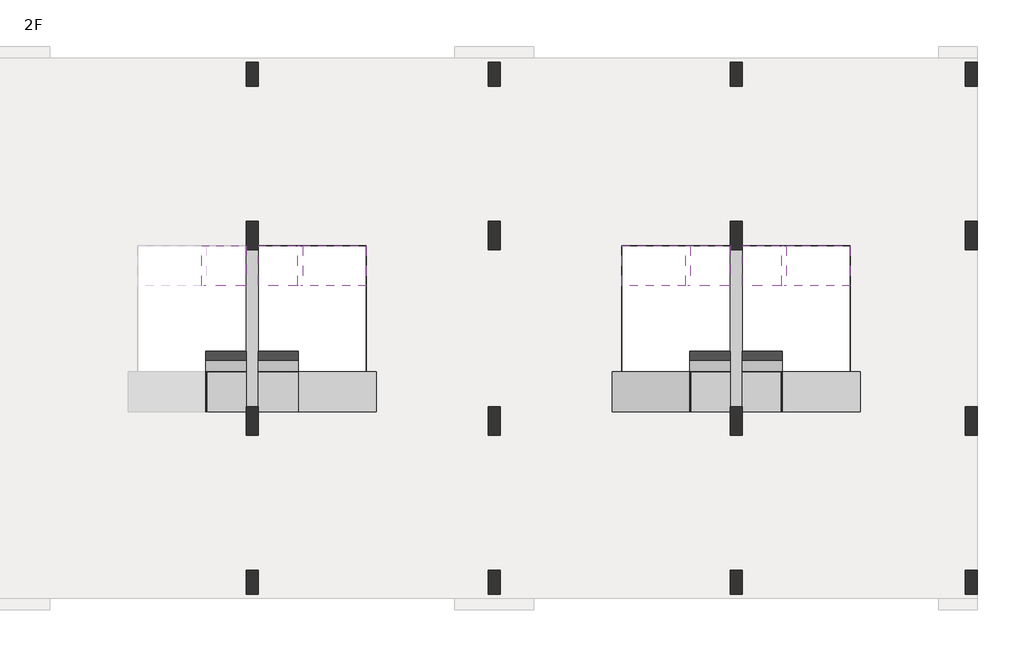
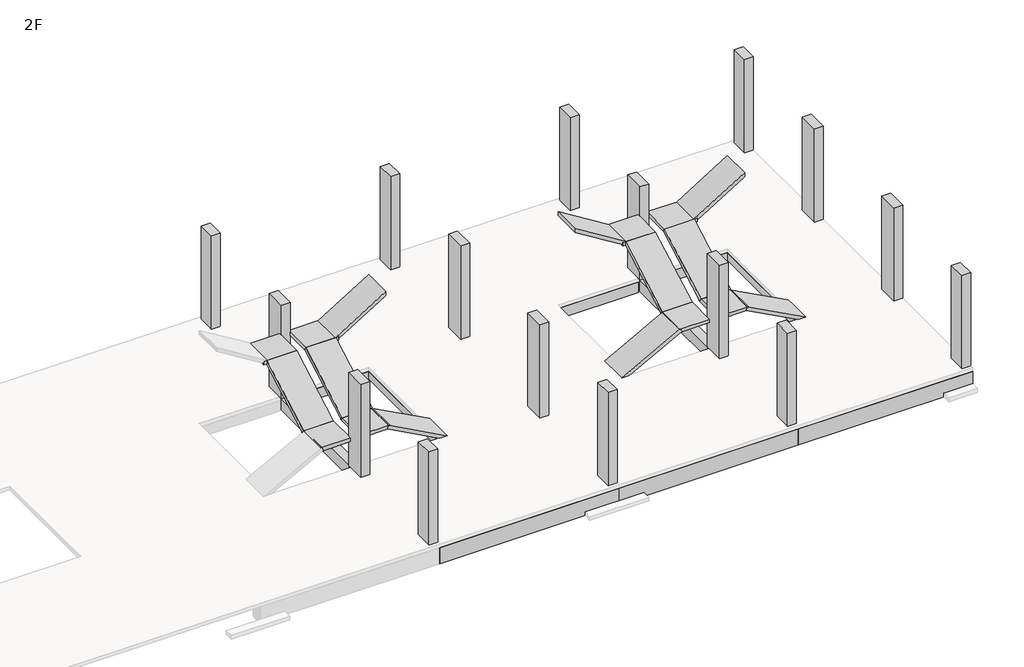
# One storey, part 2 of 2: 45 beams, 16 columns.
"""IFC4 building model written with IfcOpenShell, lengths in millimetres."""

from ifc_helpers import new_model, si_unit, frame, origin, place, context, project, spatial, polyline, outline, extrude, faceted_brep, element, save

model = new_model("IFC4")

# Units and contexts
model_context = context("Model", 3, world=origin())
ifc_project = project(units=[si_unit("LENGTHUNIT", "METRE", prefix="MILLI")], contexts=[model_context])

# Site, building, storey
site = spatial("IfcSite", under=ifc_project)
building = spatial("IfcBuilding", under=site)
storey = spatial("IfcBuildingStorey", under=building, Name="2F", Elevation=4030.0)

# Beams
placement = place(None, origin())
element("IfcBeam", 1, ObjectType="M_Concrete-Rectangular Beam : 1000x120", at=placement, inside=storey, context=model_context, shape_type="Brep", body=[
    faceted_brep([(16700.0000058, 7550.0000002, 6280.0), (17700.0000058, 7550.0000002, 6280.0), (17700.0000058, 7609.0063595, 6175.5095719), (16700.0000058, 7609.0063595, 6175.5095719), (16700.0000058, 5424.9999998, 5080.0), (16700.0000058, 5484.0063591, 4975.5095719), (17700.0000058, 5484.0063591, 4975.5095719), (17700.0000058, 5424.9999998, 5080.0), (17700.0000058, 5524.9999998, 4998.6589219), (17700.0000058, 7581.5414925, 6160.0), (16700.0000058, 5524.9999998, 4998.6589219), (16700.0000058, 7581.5414925, 6160.0)], [[[0, 1, 2, 3]], [[4, 5, 6, 7]], [[1, 0, 4, 7]], [[2, 1, 7, 6, 8, 9]], [[3, 2, 9, 8, 6, 5, 10, 11]], [[0, 3, 11, 10, 5, 4]]]),
])
element("IfcBeam", 2, ObjectType="M_Concrete-Rectangular Beam : 1000x120", at=placement, inside=storey, context=model_context, shape_type="Brep", body=[
    faceted_brep([(16600.0000058, 7550.0000002, 6280.0), (16600.0000058, 8550.0000002, 6280.0), (16600.0000058, 8550.0000002, 6160.0), (16600.0000058, 7550.0000002, 6160.0), (17700.0000058, 8550.0000002, 6160.0), (17700.0000058, 8550.0000002, 6280.0), (17700.0000058, 7550.0000002, 6280.0), (17700.0000058, 7609.0063595, 6175.5095719), (17700.0000058, 7581.5414925, 6160.0), (16700.0000058, 7550.0000002, 6280.0), (16700.0000058, 7581.5414925, 6160.0), (16700.0000058, 7550.0000002, 6160.0), (16700.0000058, 7609.0063595, 6175.5095719)], [[[0, 1, 2, 3]], [[4, 5, 6, 7, 8]], [[1, 0, 9, 6, 5]], [[2, 1, 5, 4]], [[3, 2, 4, 8, 10, 11]], [[0, 3, 11, 9]], [[12, 7, 6, 9]], [[7, 12, 10, 8]], [[12, 9, 11, 10]]]),
])
element("IfcBeam", 3, ObjectType="M_Concrete-Rectangular Beam : 1000x120", at=placement, inside=storey, context=model_context, shape_type="Brep", body=[
    faceted_brep([(17700.0000058, 5524.9999998, 4960.0), (16700.0000058, 5524.9999998, 4960.0), (16700.0000058, 5524.9999998, 4998.6589219), (17700.0000058, 5524.9999998, 4998.6589219), (17700.0000058, 4424.9999998, 4960.0), (17700.0000058, 4424.9999998, 5080.0), (16730.4772117, 4424.9999998, 5080.0), (16787.1330628, 4424.9999998, 4974.2166623), (16760.588832, 4424.9999998, 4960.0), (17700.0000058, 5424.9999998, 5080.0), (16700.0000058, 5424.9999998, 5080.0), (16700.0000058, 4424.9999998, 5080.0), (17700.0000058, 5484.0063591, 4975.5095719), (16760.588832, 5424.9999998, 4960.0), (16700.0000058, 5424.9999998, 4960.0), (16700.0000058, 4424.9999998, 5063.6768996), (16700.0000058, 5484.0063591, 4975.5095719), (16700.0000058, 5424.9999998, 5063.6768996), (16730.4772117, 5424.9999998, 5080.0), (16787.1330628, 5424.9999998, 4974.2166623)], [[[0, 1, 2, 3]], [[4, 5, 6, 7, 8]], [[6, 5, 9, 10, 11]], [[5, 4, 0, 3, 12, 9]], [[1, 0, 4, 8, 13, 14]], [[15, 11, 10, 16, 2, 1, 14, 17]], [[6, 18, 19, 7]], [[18, 6, 15, 17]], [[7, 19, 13, 8]], [[19, 18, 17, 14, 13]], [[11, 15, 6]], [[12, 16, 10, 9]], [[16, 12, 3, 2]]]),
])
element("IfcBeam", 4, ObjectType="M_Concrete-Rectangular Beam : 1000x120", at=placement, inside=storey, context=model_context, shape_type="Brep", body=[
    faceted_brep([(18969.5227998, 4424.9999998, 5080.0), (18969.5227998, 5424.9999998, 5080.0), (18912.8669488, 5424.9999998, 4974.2166623), (18912.8669488, 4424.9999998, 4974.2166623), (19000.0000058, 4424.9999998, 5063.6768996), (20930.0000065, 4424.9999998, 4030.0), (20930.0000065, 5424.9999998, 4030.0), (19000.0000058, 5424.9999998, 5063.6768996), (18939.4111796, 4424.9999998, 4960.0), (20675.8338483, 4424.9999998, 4030.0), (18939.4111796, 5424.9999998, 4960.0), (20680.0000058, 5424.9999998, 4027.7686732), (20680.0000058, 4449.9999998, 4027.7686732), (20675.8338483, 4449.9999998, 4030.0), (20680.0000058, 5424.9999998, 4030.0), (20680.0000058, 4449.9999998, 4030.0)], [[[0, 1, 2, 3]], [[1, 0, 4, 5, 6, 7]], [[0, 3, 8, 9, 5, 4]], [[3, 2, 10, 11, 12, 13, 9, 8]], [[2, 1, 7, 6, 14, 11, 10]], [[14, 6, 5, 9, 13, 15]], [[11, 14, 15, 12]], [[15, 13, 12]]]),
])
element("IfcBeam", 5, ObjectType="M_Concrete-Rectangular Beam : 1000x120", at=placement, inside=storey, context=model_context, shape_type="Brep", body=[
    faceted_brep([(19000.0000058, 7550.0000002, 6280.0), (19000.0000058, 7609.0063595, 6175.5095719), (18000.0000058, 7609.0063595, 6175.5095719), (18000.0000058, 7550.0000002, 6280.0), (19000.0000058, 5424.9999998, 5080.0), (18000.0000058, 5424.9999998, 5080.0), (18000.0000058, 5484.0063591, 4975.5095719), (19000.0000058, 5484.0063591, 4975.5095719), (18000.0000058, 7581.5414925, 6160.0), (18000.0000058, 5524.9999998, 4998.6589219), (19000.0000058, 7581.5414925, 6160.0), (19000.0000058, 5524.9999998, 4998.6589219)], [[[0, 1, 2, 3]], [[4, 5, 6, 7]], [[3, 5, 4, 0]], [[2, 8, 9, 6, 5, 3]], [[1, 10, 11, 7, 6, 9, 8, 2]], [[0, 4, 7, 11, 10, 1]]]),
])
element("IfcBeam", 6, ObjectType="M_Concrete-Rectangular Beam : 1000x120", at=placement, inside=storey, context=model_context, shape_type="Brep", body=[
    faceted_brep([(19100.0000058, 8550.0000002, 6280.0), (19100.0000058, 7550.0000002, 6280.0), (19100.0000058, 7550.0000002, 6160.0), (19100.0000058, 8550.0000002, 6160.0), (18000.0000058, 8550.0000002, 6280.0), (18000.0000058, 8550.0000002, 6160.0), (18000.0000058, 7581.5414925, 6160.0), (18000.0000058, 7609.0063595, 6175.5095719), (18000.0000058, 7550.0000002, 6280.0), (19000.0000058, 7550.0000002, 6280.0), (19000.0000058, 7550.0000002, 6160.0), (19000.0000058, 7581.5414925, 6160.0), (19000.0000058, 7609.0063595, 6175.5095719)], [[[0, 1, 2, 3]], [[4, 5, 6, 7, 8]], [[1, 0, 4, 8, 9]], [[0, 3, 5, 4]], [[3, 2, 10, 11, 6, 5]], [[2, 1, 9, 10]], [[12, 9, 8, 7]], [[12, 7, 6, 11]], [[9, 12, 11, 10]]]),
])
element("IfcBeam", 7, ObjectType="M_Concrete-Rectangular Beam : 1000x120", at=placement, inside=storey, context=model_context, shape_type="Brep", body=[
    faceted_brep([(18984.2496976, 7549.9999993, 6280.0), (20680.0000464, 7549.9999993, 7330.0), (20680.0000058, 8549.9999993, 7329.9999748), (18984.2496976, 8549.9999993, 6280.0), (20680.0000058, 8549.9999993, 7188.8582241), (19100.0000058, 8549.9999993, 6210.5302519), (19100.0000058, 8549.9999993, 6280.0), (19100.0000058, 7549.9999993, 6210.5302519), (20680.0000058, 7549.9999993, 7188.8582241), (19000.0000058, 7549.9999993, 6280.0), (19100.0000058, 7549.9999993, 6280.0)], [[[0, 1, 2, 3]], [[3, 2, 4, 5, 6]], [[7, 5, 4, 8]], [[1, 0, 9, 10, 7, 8]], [[10, 6, 5, 7]], [[6, 10, 9, 0, 3]], [[2, 1, 8, 4]]]),
])
element("IfcBeam", 8, ObjectType="M_Concrete-Rectangular Beam : 1000x120", at=placement, inside=storey, context=model_context, shape_type="Brep", body=[
    faceted_brep([(19000.0000058, 5524.9999998, 4960.0), (18000.0000058, 5524.9999998, 4960.0), (18000.0000058, 5524.9999998, 4998.6589219), (19000.0000058, 5524.9999998, 4998.6589219), (18000.0000058, 4424.9999998, 5080.0), (18000.0000058, 4424.9999998, 4960.0), (18939.4111796, 4424.9999998, 4960.0), (18912.8669488, 4424.9999998, 4974.2166623), (18969.5227998, 4424.9999998, 5080.0), (19000.0000058, 4424.9999998, 5080.0), (19000.0000058, 5424.9999998, 5080.0), (18000.0000058, 5424.9999998, 5080.0), (18000.0000058, 5484.0063591, 4975.5095719), (19000.0000058, 5424.9999998, 4960.0), (18939.4111796, 5424.9999998, 4960.0), (19000.0000058, 4424.9999998, 5063.6768996), (19000.0000058, 5424.9999998, 5063.6768996), (19000.0000058, 5484.0063591, 4975.5095719), (18969.5227998, 5424.9999998, 5080.0), (18912.8669488, 5424.9999998, 4974.2166623)], [[[0, 1, 2, 3]], [[4, 5, 6, 7, 8]], [[8, 9, 10, 11, 4]], [[5, 4, 11, 12, 2, 1]], [[1, 0, 13, 14, 6, 5]], [[9, 15, 16, 13, 0, 3, 17, 10]], [[18, 8, 7, 19]], [[8, 18, 16, 15]], [[19, 7, 6, 14]], [[18, 19, 14, 13, 16]], [[15, 9, 8]], [[17, 12, 11, 10]], [[12, 17, 3, 2]]]),
])
element("IfcBeam", 9, ObjectType="M_Concrete-Rectangular Beam : 1000x120", at=placement, inside=storey, context=model_context, shape_type="Brep", body=[
    faceted_brep([(28730.4772098, 5424.9999998, 5080.0), (28730.4772098, 4424.9999998, 5080.0), (28787.1330609, 4424.9999998, 4974.2166623), (28787.1330609, 5424.9999998, 4974.2166623), (28700.0000039, 5424.9999998, 5063.6768996), (26770.0000031, 5424.9999998, 4030.0), (26770.0000031, 4424.9999998, 4030.0), (28700.0000039, 4424.9999998, 5063.6768996), (27024.1661613, 4424.9999998, 4030.0), (28760.5888301, 4424.9999998, 4960.0), (27024.1661613, 4449.9999998, 4030.0), (27020.000004, 4449.9999998, 4027.7686733), (27020.000004, 5424.9999998, 4027.7686733), (28760.5888301, 5424.9999998, 4960.0), (27020.000004, 5424.9999998, 4030.0), (27020.000004, 4449.9999998, 4030.0)], [[[0, 1, 2, 3]], [[1, 0, 4, 5, 6, 7]], [[2, 1, 7, 6, 8, 9]], [[3, 2, 9, 8, 10, 11, 12, 13]], [[0, 3, 13, 12, 14, 5, 4]], [[5, 14, 15, 10, 8, 6]], [[14, 12, 11, 15]], [[10, 15, 11]]]),
])
element("IfcBeam", 10, ObjectType="M_Concrete-Rectangular Beam : 1000x120", at=placement, inside=storey, context=model_context, shape_type="Brep", body=[
    faceted_brep([(28700.0000039, 7550.0000002, 6280.0), (29700.0000039, 7550.0000002, 6280.0), (29700.0000039, 7609.0063595, 6175.5095719), (28700.0000039, 7609.0063595, 6175.5095719), (28700.0000039, 5424.9999998, 5080.0), (28700.0000039, 5484.0063591, 4975.5095719), (29700.0000039, 5484.0063591, 4975.5095719), (29700.0000039, 5424.9999998, 5080.0), (29700.0000039, 5524.9999998, 4998.6589219), (29700.0000039, 7581.5414925, 6160.0), (28700.0000039, 5524.9999998, 4998.6589219), (28700.0000039, 7581.5414925, 6160.0)], [[[0, 1, 2, 3]], [[4, 5, 6, 7]], [[1, 0, 4, 7]], [[2, 1, 7, 6, 8, 9]], [[3, 2, 9, 8, 6, 5, 10, 11]], [[0, 3, 11, 10, 5, 4]]]),
])
element("IfcBeam", 11, ObjectType="M_Concrete-Rectangular Beam : 1000x120", at=placement, inside=storey, context=model_context, shape_type="Brep", body=[
    faceted_brep([(28600.0000039, 7550.0000002, 6280.0), (28600.0000039, 8550.0000002, 6280.0), (28600.0000039, 8550.0000002, 6160.0), (28600.0000039, 7550.0000002, 6160.0), (29700.0000039, 8550.0000002, 6160.0), (29700.0000039, 8550.0000002, 6280.0), (29700.0000039, 7550.0000002, 6280.0), (29700.0000039, 7609.0063595, 6175.5095719), (29700.0000039, 7581.5414925, 6160.0), (28700.0000039, 7550.0000002, 6280.0), (28700.0000039, 7581.5414925, 6160.0), (28700.0000039, 7550.0000002, 6160.0), (28700.0000039, 7609.0063595, 6175.5095719)], [[[0, 1, 2, 3]], [[4, 5, 6, 7, 8]], [[1, 0, 9, 6, 5]], [[2, 1, 5, 4]], [[3, 2, 4, 8, 10, 11]], [[0, 3, 11, 9]], [[12, 7, 6, 9]], [[7, 12, 10, 8]], [[12, 9, 11, 10]]]),
])
element("IfcBeam", 12, ObjectType="M_Concrete-Rectangular Beam : 1000x120", at=placement, inside=storey, context=model_context, shape_type="Brep", body=[
    faceted_brep([(27019.9999632, 7549.9999993, 7330.0), (28715.750312, 7549.9999993, 6280.0), (28715.750312, 8549.9999993, 6280.0), (27019.9999632, 8549.9999993, 7330.0), (28600.0000039, 8549.9999993, 6280.0), (28600.0000039, 8549.9999993, 6210.5302519), (27020.000004, 8549.9999993, 7188.8582239), (28600.0000039, 7549.9999993, 6210.5302519), (27020.000004, 7549.9999993, 7188.8582239), (28600.0000039, 7549.9999993, 6280.0), (28700.0000039, 7549.9999993, 6280.0)], [[[0, 1, 2, 3]], [[3, 2, 4, 5, 6]], [[5, 7, 8, 6]], [[1, 0, 8, 7, 9, 10]], [[4, 9, 7, 5]], [[9, 4, 2, 1, 10]], [[0, 3, 6, 8]]]),
])
element("IfcBeam", 13, ObjectType="M_Concrete-Rectangular Beam : 1000x120", at=placement, inside=storey, context=model_context, shape_type="Brep", body=[
    faceted_brep([(29700.0000039, 5524.9999998, 4960.0), (28700.0000039, 5524.9999998, 4960.0), (28700.0000039, 5524.9999998, 4998.6589219), (29700.0000039, 5524.9999998, 4998.6589219), (29700.0000039, 4424.9999998, 4960.0), (29700.0000039, 4424.9999998, 5080.0), (28730.4772098, 4424.9999998, 5080.0), (28787.1330609, 4424.9999998, 4974.2166623), (28760.5888301, 4424.9999998, 4960.0), (29700.0000039, 5424.9999998, 5080.0), (28700.0000039, 5424.9999998, 5080.0), (28700.0000039, 4424.9999998, 5080.0), (29700.0000039, 5484.0063591, 4975.5095719), (28760.5888301, 5424.9999998, 4960.0), (28700.0000039, 5424.9999998, 4960.0), (28700.0000039, 4424.9999998, 5063.6768996), (28700.0000039, 5484.0063591, 4975.5095719), (28700.0000039, 5424.9999998, 5063.6768996), (28730.4772098, 5424.9999998, 5080.0), (28787.1330609, 5424.9999998, 4974.2166623)], [[[0, 1, 2, 3]], [[4, 5, 6, 7, 8]], [[6, 5, 9, 10, 11]], [[5, 4, 0, 3, 12, 9]], [[1, 0, 4, 8, 13, 14]], [[15, 11, 10, 16, 2, 1, 14, 17]], [[6, 18, 19, 7]], [[18, 6, 15, 17]], [[7, 19, 13, 8]], [[19, 18, 17, 14, 13]], [[11, 15, 6]], [[12, 16, 10, 9]], [[16, 12, 3, 2]]]),
])
element("IfcBeam", 14, ObjectType="M_Concrete-Rectangular Beam : 1000x120", at=placement, inside=storey, context=model_context, shape_type="Brep", body=[
    faceted_brep([(30969.5227979, 4424.9999998, 5080.0), (30969.5227979, 5424.9999998, 5080.0), (30912.8669468, 5424.9999998, 4974.2166623), (30912.8669468, 4424.9999998, 4974.2166623), (31000.0000039, 4424.9999998, 5063.6768996), (32930.0000046, 4424.9999998, 4030.0), (32930.0000046, 5424.9999998, 4030.0), (31000.0000039, 5424.9999998, 5063.6768996), (30939.4111776, 4424.9999998, 4960.0), (32675.8338464, 4424.9999998, 4030.0), (30939.4111776, 5424.9999998, 4960.0), (32680.0000108, 5424.9999998, 4027.7686695), (32680.0000108, 4449.9999998, 4027.7686695), (32675.8338464, 4449.9999998, 4030.0), (32680.0000108, 5424.9999998, 4030.0), (32680.0000108, 4449.9999998, 4030.0)], [[[0, 1, 2, 3]], [[1, 0, 4, 5, 6, 7]], [[0, 3, 8, 9, 5, 4]], [[3, 2, 10, 11, 12, 13, 9, 8]], [[2, 1, 7, 6, 14, 11, 10]], [[14, 6, 5, 9, 13, 15]], [[11, 14, 15, 12]], [[15, 13, 12]]]),
])
element("IfcBeam", 15, ObjectType="M_Concrete-Rectangular Beam : 1000x120", at=placement, inside=storey, context=model_context, shape_type="Brep", body=[
    faceted_brep([(31000.0000039, 7550.0000002, 6280.0), (31000.0000039, 7609.0063595, 6175.5095719), (30000.0000039, 7609.0063595, 6175.5095719), (30000.0000039, 7550.0000002, 6280.0), (31000.0000039, 5424.9999998, 5080.0), (30000.0000039, 5424.9999998, 5080.0), (30000.0000039, 5484.0063591, 4975.5095719), (31000.0000039, 5484.0063591, 4975.5095719), (30000.0000039, 7581.5414925, 6160.0), (30000.0000039, 5524.9999998, 4998.6589219), (31000.0000039, 7581.5414925, 6160.0), (31000.0000039, 5524.9999998, 4998.6589219)], [[[0, 1, 2, 3]], [[4, 5, 6, 7]], [[3, 5, 4, 0]], [[2, 8, 9, 6, 5, 3]], [[1, 10, 11, 7, 6, 9, 8, 2]], [[0, 4, 7, 11, 10, 1]]]),
])
element("IfcBeam", 16, ObjectType="M_Concrete-Rectangular Beam : 1000x120", at=placement, inside=storey, context=model_context, shape_type="Brep", body=[
    faceted_brep([(31100.0000039, 8550.0000002, 6280.0), (31100.0000039, 7550.0000002, 6280.0), (31100.0000039, 7550.0000002, 6160.0), (31100.0000039, 8550.0000002, 6160.0), (30000.0000039, 8550.0000002, 6280.0), (30000.0000039, 8550.0000002, 6160.0), (30000.0000039, 7581.5414925, 6160.0), (30000.0000039, 7609.0063595, 6175.5095719), (30000.0000039, 7550.0000002, 6280.0), (31000.0000039, 7550.0000002, 6280.0), (31000.0000039, 7550.0000002, 6160.0), (31000.0000039, 7581.5414925, 6160.0), (31000.0000039, 7609.0063595, 6175.5095719)], [[[0, 1, 2, 3]], [[4, 5, 6, 7, 8]], [[1, 0, 4, 8, 9]], [[0, 3, 5, 4]], [[3, 2, 10, 11, 6, 5]], [[2, 1, 9, 10]], [[12, 9, 8, 7]], [[12, 7, 6, 11]], [[9, 12, 11, 10]]]),
])
element("IfcBeam", 17, ObjectType="M_Concrete-Rectangular Beam : 1000x120", at=placement, inside=storey, context=model_context, shape_type="Brep", body=[
    faceted_brep([(30984.2496957, 7549.9999993, 6280.0), (32680.0000445, 7549.9999993, 7330.0), (32680.0000108, 8549.9999993, 7329.9999791), (30984.2496957, 8549.9999993, 6280.0), (32680.0000108, 8549.9999993, 7188.8582284), (31100.0000039, 8549.9999993, 6210.5302519), (31100.0000039, 8549.9999993, 6280.0), (31100.0000039, 7549.9999993, 6210.5302519), (32680.0000108, 7549.9999993, 7188.8582284), (31000.0000039, 7549.9999993, 6280.0), (31100.0000039, 7549.9999993, 6280.0)], [[[0, 1, 2, 3]], [[3, 2, 4, 5, 6]], [[7, 5, 4, 8]], [[1, 0, 9, 10, 7, 8]], [[10, 6, 5, 7]], [[6, 10, 9, 0, 3]], [[2, 1, 8, 4]]]),
])
element("IfcBeam", 18, ObjectType="M_Concrete-Rectangular Beam : 1000x120", at=placement, inside=storey, context=model_context, shape_type="Brep", body=[
    faceted_brep([(31000.0000039, 5524.9999998, 4960.0), (30000.0000039, 5524.9999998, 4960.0), (30000.0000039, 5524.9999998, 4998.6589219), (31000.0000039, 5524.9999998, 4998.6589219), (30000.0000039, 4424.9999998, 5080.0), (30000.0000039, 4424.9999998, 4960.0), (30939.4111776, 4424.9999998, 4960.0), (30912.8669468, 4424.9999998, 4974.2166623), (30969.5227979, 4424.9999998, 5080.0), (31000.0000039, 4424.9999998, 5080.0), (31000.0000039, 5424.9999998, 5080.0), (30000.0000039, 5424.9999998, 5080.0), (30000.0000039, 5484.0063591, 4975.5095719), (31000.0000039, 5424.9999998, 4960.0), (30939.4111776, 5424.9999998, 4960.0), (31000.0000039, 4424.9999998, 5063.6768996), (31000.0000039, 5424.9999998, 5063.6768996), (31000.0000039, 5484.0063591, 4975.5095719), (30969.5227979, 5424.9999998, 5080.0), (30912.8669468, 5424.9999998, 4974.2166623)], [[[0, 1, 2, 3]], [[4, 5, 6, 7, 8]], [[8, 9, 10, 11, 4]], [[5, 4, 11, 12, 2, 1]], [[1, 0, 13, 14, 6, 5]], [[9, 15, 16, 13, 0, 3, 17, 10]], [[18, 8, 7, 19]], [[8, 18, 16, 15]], [[19, 7, 6, 14]], [[18, 19, 14, 13, 16]], [[15, 9, 8]], [[17, 12, 11, 10]], [[12, 17, 3, 2]]]),
])
element("IfcBeam", 19, ObjectType="M_Concrete-Rectangular Beam : 250x400", at=placement, inside=storey, context=model_context, shape_type="Brep", body=[
    faceted_brep([(32930.0000108, 4449.9999998, 3630.0), (32930.0000108, 8549.9999993, 3630.0), (32930.0000108, 8549.9999993, 3900.0), (32930.0000108, 4449.9999998, 3900.0), (32680.0000108, 8549.9999993, 3630.0), (32680.0000108, 4449.9999998, 3630.0), (32680.0000108, 4449.9999998, 3900.0), (32680.0000108, 8549.9999993, 3900.0), (32680.0000108, 8549.9999993, 3881.8224584)], [[[0, 1, 2, 3]], [[4, 1, 0, 5]], [[4, 5, 6, 7, 8]], [[1, 4, 8, 7, 2]], [[5, 0, 3, 6]], [[3, 2, 7, 6]]]),
])
element("IfcBeam", 20, ObjectType="M_Concrete-Rectangular Beam : 250x400", at=placement, inside=storey, context=model_context, shape_type="Brep", body=[
    faceted_brep([(20680.0000058, 8549.9999993, 3630.0), (20680.0000058, 4449.9999998, 3630.0), (20680.0000058, 4449.9999998, 3900.0), (20680.0000058, 8549.9999993, 3900.0), (20680.0000058, 8549.9999993, 3881.8224534), (20930.0000058, 8549.9999993, 3630.0), (20930.0000058, 4449.9999998, 3630.0), (20930.0000058, 8549.9999993, 3900.0), (20930.0000058, 4449.9999998, 3900.0)], [[[0, 1, 2, 3, 4]], [[0, 5, 6, 1]], [[6, 5, 7, 8]], [[5, 0, 4, 3, 7]], [[1, 6, 8, 2]], [[3, 2, 8, 7]]]),
])
element("IfcBeam", 21, ObjectType="M_Concrete-Rectangular Beam : 250x400", at=placement, inside=storey, context=model_context, shape_type="Brep", body=[
    faceted_brep([(27020.000004, 4449.9999998, 3630.0), (27020.000004, 8549.9999993, 3630.0), (27020.000004, 8549.9999993, 3881.8224532), (27020.000004, 8549.9999993, 3900.0), (27020.000004, 4449.9999998, 3900.0), (26770.000004, 8549.9999993, 3630.0), (26770.000004, 4449.9999998, 3630.0), (26770.000004, 4449.9999998, 3900.0), (26770.000004, 8549.9999993, 3900.0)], [[[0, 1, 2, 3, 4]], [[5, 1, 0, 6]], [[5, 6, 7, 8]], [[1, 5, 8, 3, 2]], [[6, 0, 4, 7]], [[4, 3, 8, 7]]]),
])
element("IfcBeam", 22, ObjectType="M_Concrete-Rectangular Beam : 300x400", at=placement, inside=storey, context=model_context, shape_type="SweptSolid", body=[
    extrude(outline(polyline([(18000.0000046, 9150.0), (17700.0000046, 9150.0), (17700.0000046, 12500.0000003), (18000.0000046, 12500.0000003), (18000.0000046, 9150.0)])), frame((0.0, 0.0, 3630.0), z_axis=(0.0, 0.0, 1.0), x_axis=(1.0, 0.0, 0.0)), (0.0, 0.0, 1.0), 270.0),
])
element("IfcBeam", 23, ObjectType="M_Concrete-Rectangular Beam : 300x400", at=placement, inside=storey, context=model_context, shape_type="SweptSolid", body=[
    extrude(outline(polyline([(18000.0000046, 4550.0000002), (17700.0000046, 4550.0000002), (17700.0000046, 8449.9985388), (18000.0000046, 8449.9985388), (18000.0000046, 4550.0000002)])), frame((0.0, 0.0, 3630.0), z_axis=(0.0, 0.0, 1.0), x_axis=(1.0, 0.0, 0.0)), (0.0, 0.0, 1.0), 400.0),
])
element("IfcBeam", 24, ObjectType="M_Concrete-Rectangular Beam : 300x400", at=placement, inside=storey, context=model_context, shape_type="SweptSolid", body=[
    extrude(outline(polyline([(18000.0000046, 499.9999998), (17700.0000046, 499.9999998), (17700.0000046, 3850.0000002), (18000.0000046, 3850.0000002), (18000.0000046, 499.9999998)])), frame((0.0, 0.0, 3630.0), z_axis=(0.0, 0.0, 1.0), x_axis=(1.0, 0.0, 0.0)), (0.0, 0.0, 1.0), 270.0),
])
element("IfcBeam", 25, ObjectType="M_Concrete-Rectangular Beam : 300x400", at=placement, inside=storey, context=model_context, shape_type="SweptSolid", body=[
    extrude(outline(polyline([(30000.0000031, 9149.9985388), (29700.0000031, 9149.9985388), (29700.0000031, 12500.0000003), (30000.0000031, 12500.0000003), (30000.0000031, 9149.9985388)])), frame((0.0, 0.0, 3630.0), z_axis=(0.0, 0.0, 1.0), x_axis=(1.0, 0.0, 0.0)), (0.0, 0.0, 1.0), 270.0),
])
element("IfcBeam", 26, ObjectType="M_Concrete-Rectangular Beam : 300x400", at=placement, inside=storey, context=model_context, shape_type="SweptSolid", body=[
    extrude(outline(polyline([(30000.0000031, 4550.0000002), (29700.0000031, 4550.0000002), (29700.0000031, 8449.9985388), (30000.0000031, 8449.9985388), (30000.0000031, 4550.0000002)])), frame((0.0, 0.0, 3630.0), z_axis=(0.0, 0.0, 1.0), x_axis=(1.0, 0.0, 0.0)), (0.0, 0.0, 1.0), 400.0),
])
element("IfcBeam", 27, ObjectType="M_Concrete-Rectangular Beam : 300x400", at=placement, inside=storey, context=model_context, shape_type="SweptSolid", body=[
    extrude(outline(polyline([(30000.0000031, 499.9999998), (29700.0000031, 499.9999998), (29700.0000031, 3850.0000002), (30000.0000031, 3850.0000002), (30000.0000031, 499.9999998)])), frame((0.0, 0.0, 3630.0), z_axis=(0.0, 0.0, 1.0), x_axis=(1.0, 0.0, 0.0)), (0.0, 0.0, 1.0), 270.0),
])
element("IfcBeam", 28, ObjectType="M_Concrete-Rectangular Beam : 300x400", at=placement, inside=storey, context=model_context, shape_type="SweptSolid", body=[
    extrude(outline(polyline([(35835.035019, 9149.9985388), (35535.035019, 9149.9985388), (35535.035019, 12500.0000003), (35835.035019, 12500.0000003), (35835.035019, 9149.9985388)])), frame((0.0, 0.0, 3630.0), z_axis=(0.0, 0.0, 1.0), x_axis=(1.0, 0.0, 0.0)), (0.0, 0.0, 1.0), 270.0),
])
element("IfcBeam", 29, ObjectType="M_Concrete-Rectangular Beam : 300x400", at=placement, inside=storey, context=model_context, shape_type="SweptSolid", body=[
    extrude(outline(polyline([(35835.035019, 4550.0000002), (35535.035019, 4550.0000002), (35535.035019, 8449.9985388), (35835.035019, 8449.9985388), (35835.035019, 4550.0000002)])), frame((0.0, 0.0, 3630.0), z_axis=(0.0, 0.0, 1.0), x_axis=(1.0, 0.0, 0.0)), (0.0, 0.0, 1.0), 270.0),
])
element("IfcBeam", 30, ObjectType="M_Concrete-Rectangular Beam : 300x400", at=placement, inside=storey, context=model_context, shape_type="SweptSolid", body=[
    extrude(outline(polyline([(35835.035019, 499.9999998), (35535.035019, 499.9999998), (35535.035019, 3850.0000002), (35835.035019, 3850.0000002), (35835.035019, 499.9999998)])), frame((0.0, 0.0, 3630.0), z_axis=(0.0, 0.0, 1.0), x_axis=(1.0, 0.0, 0.0)), (0.0, 0.0, 1.0), 270.0),
])
element("IfcBeam", 31, ObjectType="M_Concrete-Rectangular Beam : 300x400", at=placement, inside=storey, context=model_context, shape_type="SweptSolid", body=[
    extrude(outline(polyline([(24000.000004, 9149.9985388), (23700.000004, 9149.9985388), (23700.000004, 12500.0000003), (24000.000004, 12500.0000003), (24000.000004, 9149.9985388)])), frame((0.0, 0.0, 3630.0), z_axis=(0.0, 0.0, 1.0), x_axis=(1.0, 0.0, 0.0)), (0.0, 0.0, 1.0), 270.0),
])
element("IfcBeam", 32, ObjectType="M_Concrete-Rectangular Beam : 300x400", at=placement, inside=storey, context=model_context, shape_type="SweptSolid", body=[
    extrude(outline(polyline([(24000.000004, 499.9999998), (23700.000004, 499.9999998), (23700.000004, 3850.0000002), (24000.000004, 3850.0000002), (24000.000004, 499.9999998)])), frame((0.0, 0.0, 3630.0), z_axis=(0.0, 0.0, 1.0), x_axis=(1.0, 0.0, 0.0)), (0.0, 0.0, 1.0), 270.0),
])
element("IfcBeam", 33, ObjectType="M_Concrete-Rectangular Beam : 300x400", at=placement, inside=storey, context=model_context, shape_type="SweptSolid", body=[
    extrude(outline(polyline([(24000.000004, 4550.0000002), (23700.000004, 4550.0000002), (23700.000004, 8449.9985388), (24000.000004, 8449.9985388), (24000.000004, 4550.0000002)])), frame((0.0, 0.0, 3630.0), z_axis=(0.0, 0.0, 1.0), x_axis=(1.0, 0.0, 0.0)), (0.0, 0.0, 1.0), 270.0),
])
element("IfcBeam", 34, ObjectType="M_Concrete-Rectangular Beam : 300x500", at=placement, inside=storey, context=model_context, shape_type="Brep", body=[
    faceted_brep([(18000.0000058, 8549.9999993, 3530.0), (23700.0000047, 8549.9999993, 3530.0), (23700.0000047, 8549.9999993, 3900.0), (20930.0000058, 8549.9999993, 3900.0), (20680.0000058, 8549.9999993, 3900.0), (18000.0000058, 8549.9999993, 3900.0), (18000.0000058, 8849.9999993, 3530.0), (23700.0000047, 8849.9999993, 3530.0), (18000.0000058, 8849.9999993, 3900.0), (23700.0000047, 8849.9999993, 3900.0)], [[[0, 1, 2, 3, 4, 5]], [[0, 6, 7, 1]], [[7, 6, 8, 9]], [[6, 0, 5, 8]], [[1, 7, 9, 2]], [[5, 4, 3, 2, 9, 8]]]),
])
element("IfcBeam", 35, ObjectType="M_Concrete-Rectangular Beam : 300x500", at=placement, inside=storey, context=model_context, shape_type="Brep", body=[
    faceted_brep([(18000.0000058, 4149.9999998, 3530.0), (23700.0000047, 4149.9999998, 3530.0), (23700.0000047, 4149.9999998, 3900.0), (18000.0000049, 4149.9999998, 3900.0), (18000.0000058, 4449.9999998, 3530.0), (23700.0000047, 4449.9999998, 3530.0), (18000.0000049, 4449.9999998, 3900.0), (20680.0000058, 4449.9999998, 3900.0), (20930.0000058, 4449.9999998, 3900.0), (23700.0000047, 4449.9999998, 3900.0)], [[[0, 1, 2, 3]], [[0, 4, 5, 1]], [[5, 4, 6, 7, 8, 9]], [[4, 0, 3, 6]], [[1, 5, 9, 2]], [[3, 2, 9, 8, 7, 6]]]),
])
element("IfcBeam", 36, ObjectType="M_Concrete-Rectangular Beam : 300x500", at=placement, inside=storey, context=model_context, shape_type="Brep", body=[
    faceted_brep([(24000.0000047, 8549.9999993, 3530.0), (29700.0000039, 8549.9999993, 3530.0), (29700.0000039, 8549.9999993, 3900.0), (27020.000004, 8549.9999993, 3900.0), (26770.000004, 8549.9999993, 3900.0), (24000.0000047, 8549.9999993, 3900.0), (24000.0000047, 8849.9999993, 3530.0), (29700.0000039, 8849.9999993, 3530.0), (24000.0000042, 8849.9999993, 3900.0), (29700.0000039, 8849.9999993, 3900.0)], [[[0, 1, 2, 3, 4, 5]], [[0, 6, 7, 1]], [[7, 6, 8, 9]], [[6, 0, 5, 8]], [[1, 7, 9, 2]], [[5, 4, 3, 2, 9, 8]]]),
])
element("IfcBeam", 37, ObjectType="M_Concrete-Rectangular Beam : 300x500", at=placement, inside=storey, context=model_context, shape_type="Brep", body=[
    faceted_brep([(24000.0000047, 4149.9999998, 3530.0), (29700.0000039, 4149.9999998, 3530.0), (29700.0000039, 4149.9999998, 3900.0), (24000.0000042, 4149.9999998, 3900.0), (24000.0000047, 4449.9999998, 3530.0), (29700.0000039, 4449.9999998, 3530.0), (24000.0000047, 4449.9999998, 3900.0), (26770.000004, 4449.9999998, 3900.0), (27020.000004, 4449.9999998, 3900.0), (29700.0000039, 4449.9999998, 3900.0)], [[[0, 1, 2, 3]], [[0, 4, 5, 1]], [[5, 4, 6, 7, 8, 9]], [[4, 0, 3, 6]], [[1, 5, 9, 2]], [[3, 2, 9, 8, 7, 6]]]),
])
element("IfcBeam", 38, ObjectType="M_Concrete-Rectangular Beam : 300x500", at=placement, inside=storey, context=model_context, shape_type="Brep", body=[
    faceted_brep([(30000.0000039, 8549.9999993, 3530.0), (35535.035019, 8549.9999993, 3530.0), (35535.035019, 8549.9999993, 3900.0), (32930.0000108, 8549.9999993, 3900.0), (32680.0000108, 8549.9999993, 3900.0), (30000.0000039, 8549.9999993, 3900.0), (30000.0000039, 8849.9999993, 3530.0), (35535.035019, 8849.9999993, 3530.0), (30000.0000039, 8849.9999993, 3900.0), (35535.035019, 8849.9999993, 3900.0)], [[[0, 1, 2, 3, 4, 5]], [[0, 6, 7, 1]], [[7, 6, 8, 9]], [[6, 0, 5, 8]], [[1, 7, 9, 2]], [[5, 4, 3, 2, 9, 8]]]),
])
element("IfcBeam", 39, ObjectType="M_Concrete-Rectangular Beam : 300x500", at=placement, inside=storey, context=model_context, shape_type="Brep", body=[
    faceted_brep([(30000.0000039, 4149.9999998, 3530.0), (35535.035019, 4149.9999998, 3530.0), (35535.035019, 4149.9999998, 3900.0), (30000.0000033, 4149.9999998, 3900.0), (30000.0000039, 4449.9999998, 3530.0), (35535.035019, 4449.9999998, 3530.0), (30000.0000033, 4449.9999998, 3900.0), (32680.0000108, 4449.9999998, 3900.0), (32930.0000108, 4449.9999998, 3900.0), (35535.035019, 4449.9999998, 3900.0)], [[[0, 1, 2, 3]], [[0, 4, 5, 1]], [[5, 4, 6, 7, 8, 9]], [[4, 0, 3, 6]], [[1, 5, 9, 2]], [[3, 2, 9, 8, 7, 6]]]),
])
element("IfcBeam", 40, ObjectType="M_Concrete-Rectangular Beam : 400x700", at=placement, inside=storey, context=model_context, shape_type="Brep", body=[
    faceted_brep([(18000.0000046, 12799.9999993, 3330.0), (23700.0000047, 12799.9999993, 3330.0), (23700.0000047, 12799.9999993, 3900.0), (18000.0000046, 12799.9999993, 3900.0), (23700.0000047, 13100.0000003, 3330.0), (18000.0000046, 13100.0000003, 3330.0), (18000.0000046, 13199.9999993, 3330.0), (22870.0000068, 13199.9999993, 3330.0), (24000.000004, 13199.9999993, 3330.0), (24000.000004, 13100.0000003, 3330.0), (18000.0000046, 13199.9999993, 3900.0), (24000.000004, 13199.9999993, 3900.0), (24000.000004, 13199.9999993, 3460.0), (23700.0000047, 13100.0000003, 3900.0), (24000.000004, 13100.0000003, 3900.0), (18000.0000046, 13100.0000003, 3900.0)], [[[0, 1, 2, 3]], [[4, 1, 0, 5, 6, 7, 8, 9]], [[6, 10, 11, 12, 8, 7]], [[1, 4, 13, 2]], [[4, 9, 14, 13]], [[9, 8, 12, 11, 14]], [[6, 5, 0, 3, 15, 10]], [[3, 2, 13, 14, 11, 10, 15]]]),
])
element("IfcBeam", 41, ObjectType="M_Concrete-Rectangular Beam : 400x700", at=placement, inside=storey, context=model_context, shape_type="Brep", body=[
    faceted_brep([(18000.0000046, -199.999999, 3900.0), (18000.0000046, -199.999999, 3330.0), (22869.7667686, -199.999999, 3330.0), (24000.000004, -199.999999, 3330.0), (24000.000004, -199.999999, 3460.0), (24000.000004, -199.999999, 3900.0), (23700.0000047, -100.0000002, 3330.0), (24000.000004, -100.0000002, 3330.0), (18000.0000046, -100.0000002, 3330.0), (18000.0000046, 200.000001, 3330.0), (23700.0000047, 200.000001, 3330.0), (18000.0000046, 200.000001, 3900.0), (23700.0000047, 200.000001, 3900.0), (23700.0000047, -100.0000002, 3900.0), (24000.000004, -100.0000002, 3900.0), (18000.0000046, -100.0000002, 3900.0)], [[[0, 1, 2, 3, 4, 5]], [[6, 7, 3, 2, 1, 8, 9, 10]], [[10, 9, 11, 12]], [[7, 6, 13, 14]], [[6, 10, 12, 13]], [[3, 7, 14, 5, 4]], [[9, 8, 1, 0, 15, 11]], [[0, 5, 14, 13, 12, 11, 15]]]),
])
element("IfcBeam", 42, ObjectType="M_Concrete-Rectangular Beam : 400x700", at=placement, inside=storey, context=model_context, shape_type="Brep", body=[
    faceted_brep([(24000.000004, 12799.9999993, 3330.0), (29700.0000039, 12799.9999993, 3330.0), (29700.0000039, 12799.9999993, 3900.0), (24000.000004, 12799.9999993, 3900.0), (29700.0000039, 13100.0000003, 3330.0), (24000.000004, 13100.0000003, 3330.0), (24000.000004, 13199.9999993, 3330.0), (24830.0000026, 13199.9999993, 3330.0), (30000.0000031, 13199.9999993, 3330.0), (30000.0000031, 13100.0000003, 3330.0), (30000.0000031, 13199.9999993, 3900.0), (24000.000004, 13199.9999993, 3460.0), (24000.000004, 13199.9999993, 3900.0), (29700.0000039, 13100.0000003, 3900.0), (30000.0000031, 13100.0000003, 3900.0), (24000.000004, 13100.0000003, 3900.0)], [[[0, 1, 2, 3]], [[4, 1, 0, 5, 6, 7, 8, 9]], [[10, 8, 7, 6, 11, 12]], [[1, 4, 13, 2]], [[4, 9, 14, 13]], [[9, 8, 10, 14]], [[6, 5, 0, 3, 15, 12, 11]], [[3, 2, 13, 14, 10, 12, 15]]]),
])
element("IfcBeam", 43, ObjectType="M_Concrete-Rectangular Beam : 400x700", at=placement, inside=storey, context=model_context, shape_type="Brep", body=[
    faceted_brep([(30000.0000031, -199.999999, 3330.0), (30000.0000031, -199.999999, 3900.0), (24000.000004, -199.999999, 3900.0), (24000.000004, -199.999999, 3460.0), (24000.000004, -199.999999, 3330.0), (24830.000004, -199.999999, 3330.0), (29700.0000039, 200.000001, 3330.0), (29700.0000039, -100.0000002, 3330.0), (30000.0000031, -100.0000002, 3330.0), (24000.000004, -100.0000002, 3330.0), (24000.000004, 200.000001, 3330.0), (24000.000004, 200.000001, 3900.0), (29700.0000039, 200.000001, 3900.0), (29700.0000039, -100.0000002, 3900.0), (30000.0000031, -100.0000002, 3900.0), (24000.000004, -100.0000002, 3900.0)], [[[0, 1, 2, 3, 4, 5]], [[6, 7, 8, 0, 5, 4, 9, 10]], [[6, 10, 11, 12]], [[7, 6, 12, 13]], [[0, 8, 14, 1]], [[10, 9, 4, 3, 2, 15, 11]], [[8, 7, 13, 14]], [[2, 1, 14, 13, 12, 11, 15]]]),
])
element("IfcBeam", 44, ObjectType="M_Concrete-Rectangular Beam : 400x700", at=placement, inside=storey, context=model_context, shape_type="Brep", body=[
    faceted_brep([(30000.0000031, 12799.9999993, 3330.0), (35535.035019, 12799.9999993, 3330.0), (35535.035019, 12799.9999993, 3900.0), (30000.0000031, 12799.9999993, 3900.0), (35535.035019, 13100.0000003, 3330.0), (30000.0000031, 13100.0000003, 3330.0), (30000.0000031, 13199.9999993, 3330.0), (34870.0000115, 13199.9999993, 3330.0), (35835.035019, 13199.9999993, 3330.0), (35835.035019, 13100.0000003, 3330.0), (30000.0000031, 13199.9999993, 3900.0), (35835.035019, 13199.9999993, 3900.0), (35835.035019, 13199.9999993, 3460.0), (35535.035019, 13100.0000003, 3900.0), (35835.035019, 13100.0000003, 3900.0), (30000.0000031, 13100.0000003, 3900.0)], [[[0, 1, 2, 3]], [[4, 1, 0, 5, 6, 7, 8, 9]], [[6, 10, 11, 12, 8, 7]], [[1, 4, 13, 2]], [[4, 9, 14, 13]], [[9, 8, 12, 11, 14]], [[6, 5, 0, 3, 15, 10]], [[3, 2, 13, 14, 11, 10, 15]]]),
])
element("IfcBeam", 45, ObjectType="M_Concrete-Rectangular Beam : 400x700", at=placement, inside=storey, context=model_context, shape_type="Brep", body=[
    faceted_brep([(30000.0000031, -199.999999, 3900.0), (30000.0000031, -199.999999, 3330.0), (34870.0000115, -199.999999, 3330.0), (35835.035019, -199.999999, 3330.0), (35835.035019, -199.999999, 3460.0), (35835.035019, -199.999999, 3900.0), (35535.035019, 200.000001, 3330.0), (35535.035019, -100.0000002, 3330.0), (35835.035019, -100.0000002, 3330.0), (30000.0000031, -100.0000002, 3330.0), (30000.0000031, 200.000001, 3330.0), (30000.0000031, 200.000001, 3900.0), (35535.035019, 200.000001, 3900.0), (35535.035019, -100.0000002, 3900.0), (35835.035019, -100.0000002, 3900.0), (30000.0000031, -100.0000002, 3900.0)], [[[0, 1, 2, 3, 4, 5]], [[6, 7, 8, 3, 2, 1, 9, 10]], [[6, 10, 11, 12]], [[7, 6, 12, 13]], [[3, 8, 14, 5, 4]], [[10, 9, 1, 0, 15, 11]], [[8, 7, 13, 14]], [[0, 5, 14, 13, 12, 11, 15]]]),
])

# Columns
element("IfcColumn", 46, ObjectType="M_Concrete-Rectangular-Column : 300x600", at=placement, inside=storey, context=model_context, shape_type="SweptSolid", body=[
    extrude(outline(polyline([(18000.0000058, 499.9999998), (18000.0000058, -100.0000002), (17700.0000058, -100.0000002), (17700.0000058, 499.9999998), (18000.0000058, 499.9999998)])), frame((0.0, 0.0, 4030.0), z_axis=(0.0, 0.0, 1.0), x_axis=(1.0, 0.0, 0.0)), (0.0, 0.0, 1.0), 3300.0),
])
element("IfcColumn", 47, ObjectType="M_Concrete-Rectangular-Column : 300x600", at=placement, inside=storey, context=model_context, shape_type="SweptSolid", body=[
    extrude(outline(polyline([(24000.0000047, 499.9999998), (24000.0000047, -100.0000002), (23700.0000047, -100.0000002), (23700.0000047, 499.9999998), (24000.0000047, 499.9999998)])), frame((0.0, 0.0, 4030.0), z_axis=(0.0, 0.0, 1.0), x_axis=(1.0, 0.0, 0.0)), (0.0, 0.0, 1.0), 3300.0),
])
element("IfcColumn", 48, ObjectType="M_Concrete-Rectangular-Column : 300x600", at=placement, inside=storey, context=model_context, shape_type="SweptSolid", body=[
    extrude(outline(polyline([(18000.0000058, 13100.0000003), (18000.0000058, 12500.0000003), (17700.0000058, 12500.0000003), (17700.0000058, 13100.0000003), (18000.0000058, 13100.0000003)])), frame((0.0, 0.0, 4030.0), z_axis=(0.0, 0.0, 1.0), x_axis=(1.0, 0.0, 0.0)), (0.0, 0.0, 1.0), 3300.0),
])
element("IfcColumn", 49, ObjectType="M_Concrete-Rectangular-Column : 300x600", at=placement, inside=storey, context=model_context, shape_type="SweptSolid", body=[
    extrude(outline(polyline([(24000.0000047, 13100.0000003), (24000.0000047, 12500.0000003), (23700.0000047, 12500.0000003), (23700.0000047, 13100.0000003), (24000.0000047, 13100.0000003)])), frame((0.0, 0.0, 4030.0), z_axis=(0.0, 0.0, 1.0), x_axis=(1.0, 0.0, 0.0)), (0.0, 0.0, 1.0), 3300.0),
])
element("IfcColumn", 50, ObjectType="M_Concrete-Rectangular-Column : 300x600", at=placement, inside=storey, context=model_context, shape_type="SweptSolid", body=[
    extrude(outline(polyline([(30000.0000039, 499.9999998), (30000.0000039, -100.0000002), (29700.0000039, -100.0000002), (29700.0000039, 499.9999998), (30000.0000039, 499.9999998)])), frame((0.0, 0.0, 4030.0), z_axis=(0.0, 0.0, 1.0), x_axis=(1.0, 0.0, 0.0)), (0.0, 0.0, 1.0), 3300.0),
])
element("IfcColumn", 51, ObjectType="M_Concrete-Rectangular-Column : 300x600", at=placement, inside=storey, context=model_context, shape_type="SweptSolid", body=[
    extrude(outline(polyline([(30000.0000039, 13100.0000003), (30000.0000039, 12500.0000003), (29700.0000039, 12500.0000003), (29700.0000039, 13100.0000003), (30000.0000039, 13100.0000003)])), frame((0.0, 0.0, 4030.0), z_axis=(0.0, 0.0, 1.0), x_axis=(1.0, 0.0, 0.0)), (0.0, 0.0, 1.0), 3300.0),
])
element("IfcColumn", 52, ObjectType="M_Concrete-Rectangular-Column : 300x600", at=placement, inside=storey, context=model_context, shape_type="SweptSolid", body=[
    extrude(outline(polyline([(35835.035019, 499.9999998), (35835.035019, -100.0000002), (35535.035019, -100.0000002), (35535.035019, 499.9999998), (35835.035019, 499.9999998)])), frame((0.0, 0.0, 4030.0), z_axis=(0.0, 0.0, 1.0), x_axis=(1.0, 0.0, 0.0)), (0.0, 0.0, 1.0), 3300.0),
])
element("IfcColumn", 53, ObjectType="M_Concrete-Rectangular-Column : 300x600", at=placement, inside=storey, context=model_context, shape_type="SweptSolid", body=[
    extrude(outline(polyline([(35835.035019, 13100.0000003), (35835.035019, 12500.0000003), (35535.035019, 12500.0000003), (35535.035019, 13100.0000003), (35835.035019, 13100.0000003)])), frame((0.0, 0.0, 4030.0), z_axis=(0.0, 0.0, 1.0), x_axis=(1.0, 0.0, 0.0)), (0.0, 0.0, 1.0), 3300.0),
])
element("IfcColumn", 54, ObjectType="M_Concrete-Rectangular-Column : 300x700", at=placement, inside=storey, context=model_context, shape_type="SweptSolid", body=[
    extrude(outline(polyline([(18000.0000058, 4550.0000002), (18000.0000058, 3850.0000002), (17700.0000058, 3850.0000002), (17700.0000058, 4550.0000002), (18000.0000058, 4550.0000002)])), frame((0.0, 0.0, 4030.0), z_axis=(0.0, 0.0, 1.0), x_axis=(1.0, 0.0, 0.0)), (0.0, 0.0, 1.0), 3300.0),
])
element("IfcColumn", 55, ObjectType="M_Concrete-Rectangular-Column : 300x700", at=placement, inside=storey, context=model_context, shape_type="SweptSolid", body=[
    extrude(outline(polyline([(24000.0000047, 4550.0000002), (24000.0000047, 3850.0000002), (23700.0000047, 3850.0000002), (23700.0000047, 4550.0000002), (24000.0000047, 4550.0000002)])), frame((0.0, 0.0, 4030.0), z_axis=(0.0, 0.0, 1.0), x_axis=(1.0, 0.0, 0.0)), (0.0, 0.0, 1.0), 3300.0),
])
element("IfcColumn", 56, ObjectType="M_Concrete-Rectangular-Column : 300x700", at=placement, inside=storey, context=model_context, shape_type="SweptSolid", body=[
    extrude(outline(polyline([(18000.0000058, 9149.9985388), (18000.0000058, 8449.9985388), (17700.0000058, 8449.9985388), (17700.0000058, 9149.9985388), (18000.0000058, 9149.9985388)])), frame((0.0, 0.0, 4030.0), z_axis=(0.0, 0.0, 1.0), x_axis=(1.0, 0.0, 0.0)), (0.0, 0.0, 1.0), 3300.0),
])
element("IfcColumn", 57, ObjectType="M_Concrete-Rectangular-Column : 300x700", at=placement, inside=storey, context=model_context, shape_type="SweptSolid", body=[
    extrude(outline(polyline([(24000.0000047, 9149.9985388), (24000.0000047, 8449.9985388), (23700.0000047, 8449.9985388), (23700.0000047, 9149.9985388), (24000.0000047, 9149.9985388)])), frame((0.0, 0.0, 4030.0), z_axis=(0.0, 0.0, 1.0), x_axis=(1.0, 0.0, 0.0)), (0.0, 0.0, 1.0), 3300.0),
])
element("IfcColumn", 58, ObjectType="M_Concrete-Rectangular-Column : 300x700", at=placement, inside=storey, context=model_context, shape_type="SweptSolid", body=[
    extrude(outline(polyline([(30000.0000039, 4550.0000002), (30000.0000039, 3850.0000002), (29700.0000039, 3850.0000002), (29700.0000039, 4550.0000002), (30000.0000039, 4550.0000002)])), frame((0.0, 0.0, 4030.0), z_axis=(0.0, 0.0, 1.0), x_axis=(1.0, 0.0, 0.0)), (0.0, 0.0, 1.0), 3300.0),
])
element("IfcColumn", 59, ObjectType="M_Concrete-Rectangular-Column : 300x700", at=placement, inside=storey, context=model_context, shape_type="SweptSolid", body=[
    extrude(outline(polyline([(30000.0000039, 9149.9985388), (30000.0000039, 8449.9985388), (29700.0000039, 8449.9985388), (29700.0000039, 9149.9985388), (30000.0000039, 9149.9985388)])), frame((0.0, 0.0, 4030.0), z_axis=(0.0, 0.0, 1.0), x_axis=(1.0, 0.0, 0.0)), (0.0, 0.0, 1.0), 3300.0),
])
element("IfcColumn", 60, ObjectType="M_Concrete-Rectangular-Column : 300x700", at=placement, inside=storey, context=model_context, shape_type="SweptSolid", body=[
    extrude(outline(polyline([(35835.035019, 4550.0000002), (35835.035019, 3850.0000002), (35535.035019, 3850.0000002), (35535.035019, 4550.0000002), (35835.035019, 4550.0000002)])), frame((0.0, 0.0, 4030.0), z_axis=(0.0, 0.0, 1.0), x_axis=(1.0, 0.0, 0.0)), (0.0, 0.0, 1.0), 3300.0),
])
element("IfcColumn", 61, ObjectType="M_Concrete-Rectangular-Column : 300x700", at=placement, inside=storey, context=model_context, shape_type="SweptSolid", body=[
    extrude(outline(polyline([(35835.035019, 9149.9985388), (35835.035019, 8449.9985388), (35535.035019, 8449.9985388), (35535.035019, 9149.9985388), (35835.035019, 9149.9985388)])), frame((0.0, 0.0, 4030.0), z_axis=(0.0, 0.0, 1.0), x_axis=(1.0, 0.0, 0.0)), (0.0, 0.0, 1.0), 3300.0),
])

save(model, "model.ifc")

# Revit data of these elements
# Type "M_Concrete-Rectangular Beam : 1000x120"
#   Length [instance default] = 1524 mm
#   b = 1000 mm
#   h = 120 mm
#   Structural Material [instance default] = Concrete, Cast-in-Place gray
#   Assembly Code = ""
# Type "M_Concrete-Rectangular Beam : 250x400"
#   Length [instance default] = 1524 mm
#   b = 250 mm
#   h = 400 mm
#   Structural Material [instance default] = Concrete, Cast-in-Place gray
#   Assembly Code = ""
# Type "M_Concrete-Rectangular Beam : 300x400"
#   Length [instance default] = 1524 mm
#   b = 300 mm
#   h = 400 mm
#   Structural Material [instance default] = Concrete, Cast-in-Place gray
#   Assembly Code = ""
# Type "M_Concrete-Rectangular Beam : 300x500"
#   Length [instance default] = 1524 mm
#   b = 300 mm
#   h = 500 mm
#   Structural Material [instance default] = Concrete, Cast-in-Place gray
#   Assembly Code = ""
# Type "M_Concrete-Rectangular Beam : 400x700"
#   Length [instance default] = 1524 mm
#   b = 400 mm
#   h = 700 mm
#   Structural Material [instance default] = Concrete, Cast-in-Place gray
#   Assembly Code = ""
# Type "M_Concrete-Rectangular-Column : 300x600"
#   b = 300 mm
#   h = 600 mm
#   Structural Material [instance default] = Concrete, Cast-in-Place gray
# Type "M_Concrete-Rectangular-Column : 300x700"
#   b = 300 mm
#   h = 700 mm
#   Structural Material [instance default] = Concrete, Cast-in-Place gray
# Elements 1, 2, 3, 5, 6, 7, 8, 10, 11, 12, 13, 15, 16, 17, 18 (IfcBeam, "M_Concrete-Rectangular Beam : 1000x120")
#   COF_GEN__Name = "STAIR"
#   Structural Material = Concrete, Cast-in-Place gray
#   Phase Created = New Construction
#   Materials on its faces: "Concrete, Cast-in-Place gray"
# Elements 4, 9, 14 (IfcBeam, "M_Concrete-Rectangular Beam : 1000x120")
#   Comments = ""
#   COF_GEN__Name = "STAIR"
#   Structural Material = Concrete, Cast-in-Place gray
#   Phase Created = New Construction
#   Materials on its faces: "Concrete, Cast-in-Place gray"
# Elements 19, 20, 21 (IfcBeam, "M_Concrete-Rectangular Beam : 250x400")
#   Comments = ""
#   COF_CON__WorkItemNumber = "SH3-A-02F"
#   COF_GEN__Name = "DP1"
#   Structural Material = Concrete, Cast-in-Place gray
#   Phase Created = New Construction
#   Materials on its faces: "Concrete, Cast-in-Place gray"
# Elements 22, 23, 24, 25, 26, 27, 28, 29, 30, 31, 32, 33 (IfcBeam, "M_Concrete-Rectangular Beam : 300x400")
#   Comments = ""
#   COF_CON__WorkItemNumber = "SH3-A-02F"
#   COF_GEN__Name = "D3"
#   Structural Material = Concrete, Cast-in-Place gray
#   Phase Created = New Construction
#   Materials on its faces: "Concrete, Cast-in-Place gray"
# Elements 34, 35, 36, 37, 38, 39 (IfcBeam, "M_Concrete-Rectangular Beam : 300x500")
#   Comments = ""
#   COF_CON__WorkItemNumber = "SH3-A-02F"
#   COF_GEN__Name = "D2"
#   Structural Material = Concrete, Cast-in-Place gray
#   Phase Created = New Construction
#   Materials on its faces: "Concrete, Cast-in-Place gray"
# Elements 40, 41, 42, 43, 44, 45 (IfcBeam, "M_Concrete-Rectangular Beam : 400x700")
#   Comments = ""
#   COF_CON__WorkItemNumber = "SH3-A-02F"
#   COF_GEN__Name = "D1A"
#   Structural Material = Concrete, Cast-in-Place gray
#   Phase Created = New Construction
#   Materials on its faces: "Concrete, Cast-in-Place gray"
# Elements 46, 48 (IfcColumn, "M_Concrete-Rectangular-Column : 300x600")
#   Comments = ""
#   COF_CON__WorkItemNumber = "SH3-A-03F"
#   COF_GEN__Name = "C2"
#   Structural Material = Concrete, Cast-in-Place gray
#   Phase Created = New Construction
#   Materials on its faces: "Concrete, Cast-in-Place gray"
# Elements 47, 49, 50, 51, 52, 53 (IfcColumn, "M_Concrete-Rectangular-Column : 300x600")
#   Comments = ""
#   COF_CON__WorkItemNumber = "SH3-A-03F"
#   COF_GEN__Name = "C1"
#   Structural Material = Concrete, Cast-in-Place gray
#   Phase Created = New Construction
#   Materials on its faces: "Concrete, Cast-in-Place gray"
# Elements 54, 56 (IfcColumn, "M_Concrete-Rectangular-Column : 300x700")
#   Comments = ""
#   COF_CON__WorkItemNumber = "SH3-A-03F"
#   COF_GEN__Name = "C6"
#   Structural Material = Concrete, Cast-in-Place gray
#   Phase Created = New Construction
#   Materials on its faces: "Concrete, Cast-in-Place gray"
# Elements 55, 57 (IfcColumn, "M_Concrete-Rectangular-Column : 300x700")
#   Comments = ""
#   COF_CON__WorkItemNumber = "SH3-A-03F"
#   COF_GEN__Name = "C5"
#   Structural Material = Concrete, Cast-in-Place gray
#   Phase Created = New Construction
#   Materials on its faces: "Concrete, Cast-in-Place gray"
# Elements 58, 59 (IfcColumn, "M_Concrete-Rectangular-Column : 300x700")
#   Comments = ""
#   COF_CON__WorkItemNumber = "SH3-A-03F"
#   COF_GEN__Name = "C4"
#   Structural Material = Concrete, Cast-in-Place gray
#   Phase Created = New Construction
#   Materials on its faces: "Concrete, Cast-in-Place gray"
# Elements 60, 61 (IfcColumn, "M_Concrete-Rectangular-Column : 300x700")
#   Comments = ""
#   COF_CON__WorkItemNumber = "SH3-A-03F"
#   COF_GEN__Name = "C3"
#   Structural Material = Concrete, Cast-in-Place gray
#   Phase Created = New Construction
#   Materials on its faces: "Concrete, Cast-in-Place gray"
# Materials
#   "Concrete, Cast-in-Place gray": class "Concrete", colour RGB 207 208 204, transparency 0, Description = "Cast-in-place concrete", Cost = 0
